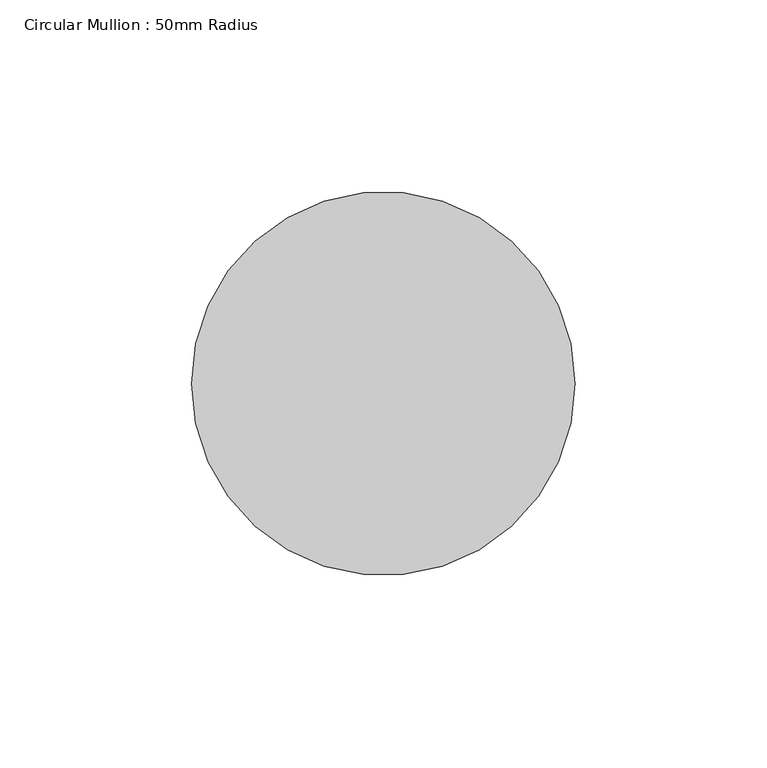
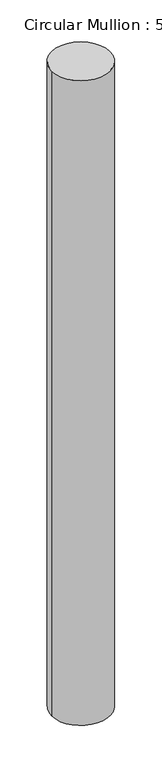
"""IFC4 building model written with IfcOpenShell, lengths in millimetres: member geometry, Circular Mullion : 50mm Radius."""

from ifc_helpers import new_model, si_unit, point, frame, origin, origin_2d, place, context, project, spatial, circle_curve, trimmed, segment, composite_curve, outline, extrude, source, transform, mapped, element, save


def circular_mullion_50mm_radius_f2383d24(model_context):
    return source(origin(), model_context, "Body", "SweptSolid", [
        extrude(outline(composite_curve([segment(trimmed(circle_curve(origin_2d(), 50.0), [point((50.0, 0.0))], [point((-50.0, 0.0))], False, "CARTESIAN"), True, "CONTINUOUS"), segment(trimmed(circle_curve(origin_2d(), 50.0), [point((-50.0, 0.0))], [point((50.0, 0.0))], False, "CARTESIAN"), True, "CONTINUOUS")], self_intersect=False)), frame((0.0, 0.0, -1167.2940359), z_axis=(0.0, 0.0, 1.0), x_axis=(1.0, 0.0, 0.0)), (0.0, 0.0, 1.0), 1167.2940359),
    ])


if __name__ == "__main__":
    model = new_model("IFC4")
    model_context = context("Model", 3, world=origin())
    ifc_project = project(units=[si_unit("LENGTHUNIT", "METRE", prefix="MILLI")], contexts=[model_context])
    site = spatial("IfcSite", under=ifc_project)
    building = spatial("IfcBuilding", under=site)
    placement = place(None, origin())
    circular_mullion_50mm_radius_shape = circular_mullion_50mm_radius_f2383d24(model_context)
    element("IfcMember", 1, ObjectType="Circular Mullion : 50mm Radius", at=placement, inside=building, context=model_context, shape_type="MappedRepresentation", body=[
        mapped(circular_mullion_50mm_radius_shape, transform((0.0, 0.0, 0.0), x_axis=(1.0, 0.0, 0.0), y_axis=(0.0, 1.0, 0.0), z_axis=(0.0, 0.0, 1.0))),
    ])
    save(model, "model.ifc")

# Revit data of these elements
# Type "Circular Mullion : 50mm Radius"
#   built-in parameter 1007350 = 0.164042 (stored number, unit not read)
# Element 1 (IfcMember, "Circular Mullion : 50mm Radius")
#   Materials on its faces: "Aluminium"
# Materials
#   "Aluminium": class "Metal", colour RGB 247 247 247, transparency 0, Description = "Aluminium 6061", Cost = 0
